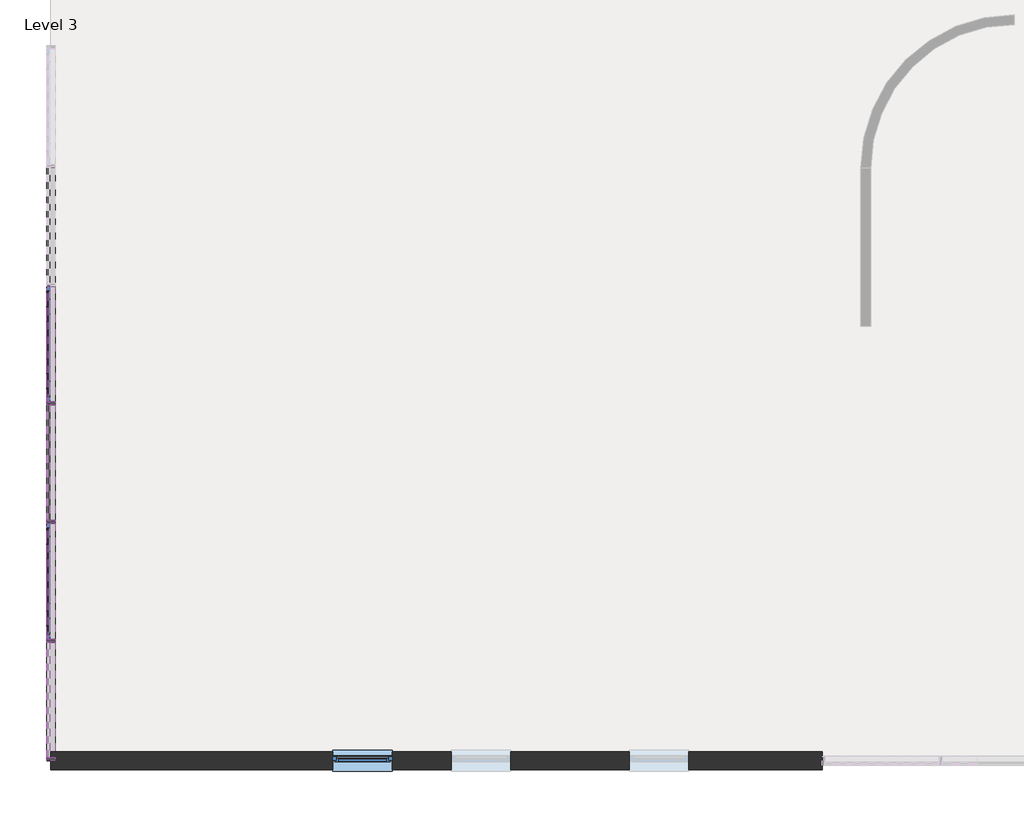
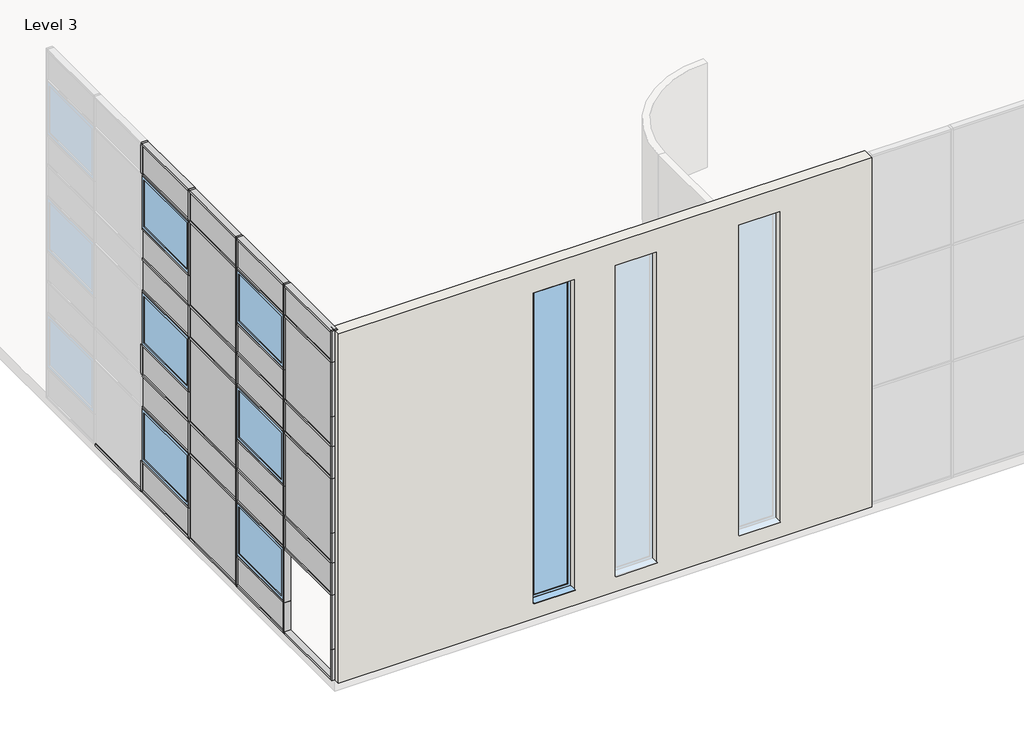
# One storey, part 1 of 5: 74 members, 23 plates, 7 windows, 1 wall.
# Revit data of these elements (continued)
# Grids (mm) (continued)
#   "2": line (-3732.003, -17149.184) -> (-3732.003, 20035.144)
#   "3": line (6267.997, -17149.184) -> (6267.997, 20035.144)
#   "4": line (16267.997, -17149.184) -> (16267.997, 20035.144)
#   "5": line (26267.997, -17149.184) -> (26267.997, 20035.144)
#   "6": line (36243.497, -17149.184) -> (36243.497, 20035.144)
#   "A": line (42039.58, 15998.758) -> (-12000.946, 15998.758)
#   "B": line (42039.58, 12998.758) -> (-12000.946, 12998.758)
#   "C": line (42039.58, 2998.758) -> (-12000.946, 2998.758)
#   "D": line (42039.58, -7001.242) -> (-12000.946, -7001.242)
#   "E": line (42039.58, -10001.242) -> (-12000.946, -10001.242)
# Type "Rectangular Mullion : 50 x 150mm"
#   built-in parameter 1007304 = 0.492126 (stored number, unit not read)
#   built-in parameter 1007301 = 0.082021 (stored number, unit not read)
#   built-in parameter 1007300 = 0.082021 (stored number, unit not read)
# Type "Exterior Wall - MPK"
#   Layers, outside or top first: 0.050 m "Metal - Panel" (function 4); 0.100 m "Insulation / Thermal Barriers - Rigid insulation" (function 3); 0.150 m "Concrete - Cast In Situ" (function 1)
# Type "M_Curtain Wall Awning : M_Curtain Wall Awning"
#   Type Mark = "20"
#   Offset = 0.075 m
#   Sash Width = 0.075 m
#   Thickness = 0.050 m
#   Define Thermal Properties by = 1
#   Glass Pane Material = Window - Glass
#   Sash Material = Metal - Aluminum
# Type "Window - Variable : Standard"
#   Type Mark = "19"
#   Operation = "SinglePanel"
#   Keynote = "16.05.01"
#   Analytic Construction = "<None>"
#   Rough Width [instance default] = 1.010 m
#   Rough Height [instance default] = 1.010 m
#   Frame Depth = 0.060 m
#   Frame Height Bottom = 0.080 m
#   Frame Height Top = 0.080 m
#   Frame Width = 0.060 m
#   Height [instance default] = 1.010 m
#   Window Inset = 0.060 m
#   Window Width = 0.060 m
#   Instalation Depth [instance default] = 0.080 m
#   Width [instance default] = 1.010 m
#   Folding Wing [instance default] = no
#   Oppening Direction Vertical [instance default] = yes
#   Oppening Direction Visibility [instance default] = no
#   Casement [instance default] = yes
#   Frame [instance default] = none
#   Glas [instance default] = none
#   Window [instance default] = none
#   Windowsill Inside [instance default] = none
#   Windowsill Outside [instance default] = none
#   Wall Closure = (empty or 0)
#   Assembly Code = ""
# Elements 1, 2, 3, 4, 5, 6, 7, 8, 9, 10, 11, 12, 13, 14, 15, 16, 17, 18, 19, 20, 21, 22, 23, 24, 25, 26, 27, 28, 29, 30, 31, 32, 33, 34, 35, 36, 37, 38, 39, 40, 41, 42, 43, 44, 45, 46, 47, 48, 49, 50, 51, 52, 53, 54, 55, 56, 57, 58, 59, 60, 61, 62, 63, 64, 65, 66, 67, 68, 69, 70, 71, 72, 73, 74 (IfcMember, "Rectangular Mullion : 50 x 150mm")
#   Phase Created = New Construction
#   Materials on its faces: "Metal - Aluminium"
# Elements 75, 76, 77, 78, 79, 80, 81, 82, 83, 84, 85, 86, 87, 88, 89, 90, 91, 92, 93, 94, 95, 96, 97 (IfcPlate, "System Panel : Glazed")
#   Phase Created = New Construction
#   Materials on its faces: "Glass"
# Element 98 (IfcWall, "Exterior Wall - MPK")
#   Top Offset = 0.000 m
#   Base Offset = 0.000 m
#   wall height = 9.000 m
#   Phase Created = New Construction
#   Base Constraint = Level 3
#   Top Constraint = Level 6
#   Materials on its faces: "Default Wall", "Concrete - Cast In Situ", "Metal - Panel"
# Elements 99, 100, 101, 102, 103, 104 (IfcWindow, "M_Curtain Wall Awning : M_Curtain Wall Awning")
#   Phase Created = New Construction
#   Materials on its faces: "Metal - Aluminum", "Window - Glass"
# Element 105 (IfcWindow, "Window - Variable : Standard")
#   Mark = "8"
#   Width = 1.000 m
#   Rough Width = 1.000 m
#   Rough Height = 8.000 m
#   Instalation Depth = 0.080 m
#   Height = 8.000 m
#   Oppening Direction Visibility = no
#   Oppening Direction Vertical = yes
#   Folding Wing = no
#   Casement = yes
#   Windowsill Outside = none
#   Windowsill Inside = none
#   Window = none
#   Glas = none
#   Frame = none
#   Phase Created = New Construction
#   Materials on its faces: "Plastic - White", "Metal _ Aluminium", "Wood - Birch", "Glass"
# Materials
#   "Metal - Panel": class "Metal", colour RGB 247 247 247, transparency 0
#   "Insulation / Thermal Barriers - Rigid insulation": class "Miscellaneous", colour RGB 127 127 127, transparency 0
#   "Concrete - Cast In Situ": class "Concrete", colour RGB 192 192 192, transparency 0
#   "Window - Glass": class "Glas", colour RGB 128 128 255, transparency 0.75
#   "Metal - Aluminum": class "Unassigned", colour RGB 247 247 247, transparency 0, Comments = "Rendering appearance not upgraded "
#   "Metal - Aluminium": class "Metal", colour RGB 247 247 247, transparency 0
#   "Glass": class "Glass", colour RGB 0 128 192, transparency 0.9
#   "Default Wall": class "Miscellaneous", colour RGB 128 128 128, transparency 0
#   "Plastic - White": class "Kunststoff", colour RGB 249 249 249, transparency 0
#   "Metal _ Aluminium": class "Metall", colour RGB 247 247 247, transparency 0
#   "Wood - Birch": class "Holz", colour RGB 213 164 103, transparency 0
